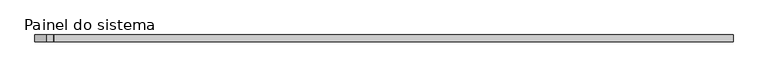
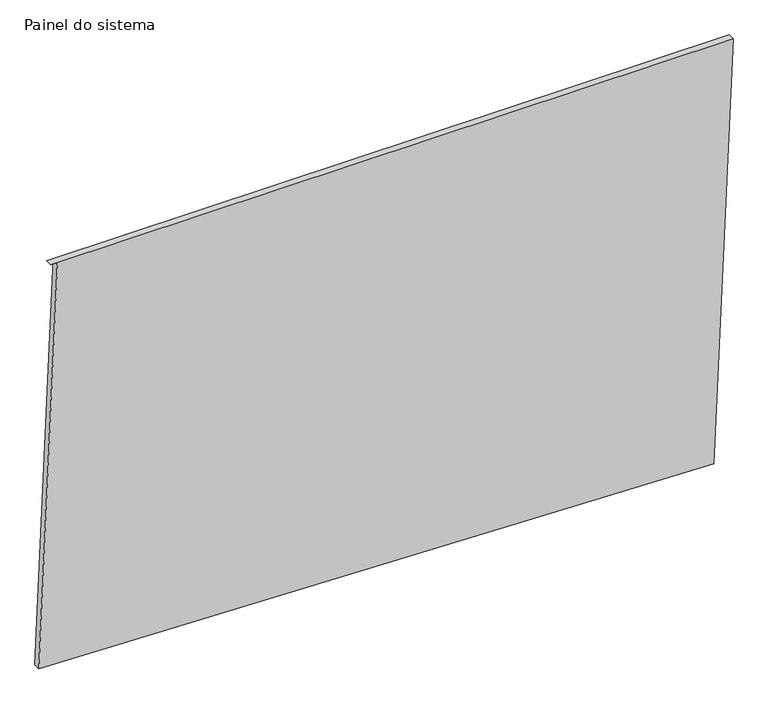
"""IFC4 building model written with IfcOpenShell, lengths in millimetres: plate geometry, Painel do sistema : Envidraçado."""

import ifcopenshell
import ifcopenshell.guid

model = None  # the IFC model being written
_history = None  # IfcOwnerHistory: only IFC2X3 demands one
_inside = {}  # id of a spatial element -> (the spatial element, [elements in it])
_under = {}  # id of a project, library or spatial element -> (it, [spatial elements below it])
_declared = {}  # id of a project -> (the project, [libraries it declares])
_typed = {}  # id of a type object -> (the type object, [elements of that type])
_made_of = {}  # id of a material, layer set ... -> (it, [elements and type objects made of it])


def new_model(schema):
    """Start an empty IFC model of exactly this schema.

    Asked for "IFC4X3", IfcOpenShell would pick the latest addendum, in which some entities
    have other attributes; the version numbers below select the first issue.
    IFC2X3 requires an IfcOwnerHistory on every rooted entity: one is made here for all.
    """
    global model, _history
    if schema == "IFC4X3":
        model = ifcopenshell.file(schema_version=(4, 3, 0, 0))
    else:
        model = ifcopenshell.file(schema=schema)
    _inside.clear()
    _under.clear()
    _declared.clear()
    _typed.clear()
    _made_of.clear()
    _history = None
    if model.schema == "IFC2X3":
        org = make("IfcOrganization", Name="unknown")
        user = make(
            "IfcPersonAndOrganization",
            ThePerson=make("IfcPerson", FamilyName="unknown"),
            TheOrganization=org,
        )
        app = make(
            "IfcApplication",
            ApplicationDeveloper=org,
            Version="unknown",
            ApplicationFullName="unknown",
            ApplicationIdentifier="unknown",
        )
        _history = make(
            "IfcOwnerHistory",
            OwningUser=user,
            OwningApplication=app,
            ChangeAction="ADDED",
            CreationDate=0,
        )
    return model


def make(cls, **values):
    """One entity of the class cls with the attributes given. An attribute that is None is left unset."""
    return model.create_entity(
        cls, **{name: value for name, value in values.items() if value is not None}
    )


def rooted(cls, **values):
    """An entity with a GlobalId (a new one), such as an element, a storey or a relation."""
    return make(cls, GlobalId=ifcopenshell.guid.new(), OwnerHistory=_history, **values)


def si_unit(unit_type, name, prefix=None):
    """IfcSIUnit, for example si_unit("LENGTHUNIT", "METRE", prefix="MILLI")."""
    return make("IfcSIUnit", UnitType=unit_type, Prefix=prefix, Name=name)


def assignment(units):
    """IfcUnitAssignment: the units of a project."""
    return None if units is None else make("IfcUnitAssignment", Units=units)


def point(xyz):
    """IfcCartesianPoint."""
    return None if xyz is None else make("IfcCartesianPoint", Coordinates=xyz)


def direction(xyz):
    """IfcDirection."""
    return None if xyz is None else make("IfcDirection", DirectionRatios=xyz)


def frame(location, z_axis=None, x_axis=None):
    """IfcAxis2Placement3D, a coordinate frame: its origin and axes. An axis left out is left unset."""
    return make(
        "IfcAxis2Placement3D",
        Location=point(location),
        Axis=direction(z_axis),
        RefDirection=direction(x_axis),
    )


def origin():
    """The frame at (0, 0, 0) with its axes left unset."""
    return frame((0.0, 0.0, 0.0))


def place(relative_to, where):
    """IfcLocalPlacement: puts the frame where relative to a parent placement (None: the world)."""
    return make(
        "IfcLocalPlacement", PlacementRelTo=relative_to, RelativePlacement=where
    )


def context(
    kind, dimensions, precision=None, world=None, true_north=None, identifier=None
):
    """IfcGeometricRepresentationContext, for example the 3D "Model" context."""
    return make(
        "IfcGeometricRepresentationContext",
        ContextIdentifier=identifier,
        ContextType=kind,
        CoordinateSpaceDimension=dimensions,
        Precision=precision,
        WorldCoordinateSystem=world,
        TrueNorth=true_north,
    )


def project(units=None, contexts=None):
    """IfcProject with its units and contexts."""
    return rooted(
        "IfcProject",
        Name="project",
        RepresentationContexts=contexts,
        UnitsInContext=assignment(units),
    )


def spatial(cls, under=None, at=None, **own):
    """A site, building, storey or space (cls), placed at a placement, below another one or the project."""
    s = rooted(cls, ObjectPlacement=at, **own)
    if under is not None:
        _under.setdefault(under.id(), (under, []))[1].append(s)
    return s


def polyline(points):
    """IfcPolyline through the points."""
    return make("IfcPolyline", Points=[point(p) for p in points])


def outline(outer, holes=None, kind="AREA"):
    """IfcArbitraryClosedProfileDef: a profile drawn as a closed curve; with holes, ...WithVoids."""
    if holes is None:
        return make("IfcArbitraryClosedProfileDef", ProfileType=kind, OuterCurve=outer)
    return make(
        "IfcArbitraryProfileDefWithVoids",
        ProfileType=kind,
        OuterCurve=outer,
        InnerCurves=holes,
    )


def extrude(swept, where, along, depth):
    """IfcExtrudedAreaSolid: the profile swept, set in the frame where, extruded along a direction by depth."""
    return make(
        "IfcExtrudedAreaSolid",
        SweptArea=swept,
        Position=where,
        ExtrudedDirection=direction(along),
        Depth=depth,
    )


def shape(context_of_items, identifier, shape_type, items):
    """IfcShapeRepresentation: the items that make up one representation, for example the "Body"."""
    return make(
        "IfcShapeRepresentation",
        ContextOfItems=context_of_items,
        RepresentationIdentifier=identifier,
        RepresentationType=shape_type,
        Items=items,
    )


def source(mapping_origin, context_of_items, identifier, shape_type, items):
    """IfcRepresentationMap: a shape defined once, which mapped items show again and again."""
    return make(
        "IfcRepresentationMap",
        MappingOrigin=mapping_origin,
        MappedRepresentation=shape(context_of_items, identifier, shape_type, items),
    )


def transform(
    local_origin,
    x_axis=None,
    y_axis=None,
    z_axis=None,
    scale=None,
    scale2=None,
    scale3=None,
    uniform=True,
):
    """IfcCartesianTransformationOperator3D, or its non-uniform kind. x_axis, y_axis, z_axis: its Axis1, 2, 3."""
    if uniform:
        return make(
            "IfcCartesianTransformationOperator3D",
            Axis1=direction(x_axis),
            Axis2=direction(y_axis),
            LocalOrigin=point(local_origin),
            Scale=scale,
            Axis3=direction(z_axis),
        )
    return make(
        "IfcCartesianTransformationOperator3DnonUniform",
        Axis1=direction(x_axis),
        Axis2=direction(y_axis),
        LocalOrigin=point(local_origin),
        Scale=scale,
        Axis3=direction(z_axis),
        Scale2=scale2,
        Scale3=scale3,
    )


def mapped(mapping_source, mapping_target):
    """IfcMappedItem: shows the shape of a source again, moved by a transform."""
    return make(
        "IfcMappedItem", MappingSource=mapping_source, MappingTarget=mapping_target
    )


def made_of(thing, what):
    """Note that an element or type object is made of a material, layer set ...; save() writes the relation."""
    if what is not None:
        _made_of.setdefault(what.id(), (what, []))[1].append(thing)
    return thing


def element(
    cls,
    number,
    at=None,
    inside=None,
    cuts=None,
    type_object=None,
    material=None,
    context=None,
    identifier="Body",
    shape_type=None,
    held_by="IfcProductDefinitionShape",
    body=None,
    shapes=None,
    **own,
):
    """One element of the class cls, such as IfcWall. Its Tag is "e" and its number.

    at: its placement. inside: the storey or other place that contains it. cuts: it is an
    opening in that element (IfcRelVoidsElement). A single representation is given by context,
    identifier, shape_type and body (its items); several are given by shapes. held_by: the class
    of the entity that holds the representations. save() writes the other relations.
    """
    e = rooted(cls, Tag="e%d" % number, ObjectPlacement=at, **own)
    if body is not None:
        shapes = [shape(context, identifier, shape_type, body)]
    if shapes is not None:
        e.Representation = make(held_by, Representations=shapes)
    if inside is not None:
        _inside.setdefault(inside.id(), (inside, []))[1].append(e)
    if cuts is not None:
        rooted(
            "IfcRelVoidsElement", RelatingBuildingElement=cuts, RelatedOpeningElement=e
        )
    if type_object is not None:
        _typed.setdefault(type_object.id(), (type_object, []))[1].append(e)
    return made_of(e, material)


def aggregate(whole, parts):
    """IfcRelAggregates: a whole, such as a stair, and the parts it consists of."""
    return rooted("IfcRelAggregates", RelatingObject=whole, RelatedObjects=parts)


def save(model, path):
    """Write the relations noted so far, then the file.

    IfcRelAggregates (storeys below a building ...), IfcRelContainedInSpatialStructure (elements
    in a storey), IfcRelDefinesByType, IfcRelAssociatesMaterial and IfcRelDeclares: one each for
    every whole, place, type object, material and project.
    """
    for whole, parts in _under.values():
        aggregate(whole, parts)
    for where, things in _inside.values():
        rooted(
            "IfcRelContainedInSpatialStructure",
            RelatedElements=things,
            RelatingStructure=where,
        )
    for kind, things in _typed.values():
        rooted("IfcRelDefinesByType", RelatedObjects=things, RelatingType=kind)
    for what, things in _made_of.values():
        rooted("IfcRelAssociatesMaterial", RelatedObjects=things, RelatingMaterial=what)
    for by, libraries in _declared.values():
        rooted("IfcRelDeclares", RelatingContext=by, RelatedDefinitions=libraries)
    model.write(path)


def painel_do_sistema_41383344(model_context):
    return source(origin(), model_context, "Body", "SweptSolid", [
        extrude(outline(polyline([(72.8211161, -1297.2364294), (0.0, 1224.626647), (1652.651399, 1297.2364294), (1652.651399, -1252.850184), (1651.5540743, -1227.874278), (72.8211161, -1297.2364294)])), frame((0.0, 24.5, 0.0), z_axis=(0.0, 1.0, 0.0), x_axis=(0.0, 0.0, 1.0)), (0.0, 0.0, 1.0), 25.0),
    ])


if __name__ == "__main__":
    model = new_model("IFC4")
    model_context = context("Model", 3, world=origin())
    ifc_project = project(units=[si_unit("LENGTHUNIT", "METRE", prefix="MILLI")], contexts=[model_context])
    site = spatial("IfcSite", under=ifc_project)
    building = spatial("IfcBuilding", under=site)
    placement = place(None, origin())
    painel_do_sistema_shape = painel_do_sistema_41383344(model_context)
    element("IfcPlate", 1, ObjectType="Painel do sistema : Envidraçado", at=placement, inside=building, context=model_context, shape_type="MappedRepresentation", body=[
        mapped(painel_do_sistema_shape, transform((0.0, 0.0, 0.0), x_axis=(1.0, 0.0, 0.0), y_axis=(0.0, 1.0, 0.0), z_axis=(0.0, 0.0, 1.0))),
    ])
    save(model, "model.ifc")

# Revit data of these elements
# Type "Painel do sistema : Envidraçado"
#   Construction Type Id = "GSP4R"
#   Analytic Construction = "Vidraça única Pilkington 1/8 pol"
#   Visual Light Transmittance = 0.9
#   Solar Heat Gain Coefficient = 0.86
#   Heat Transfer Coefficient (U) = 6.7069 W/(m²·K)
# Element 1 (IfcPlate, "Painel do sistema : Envidraçado")
#   Materials on its faces: "Vidro"
# Materials
#   "Vidro": class "Vidro", colour RGB 0 128 192, transparency 0.9, Description = "Vidro de sílica", Cost = 0
